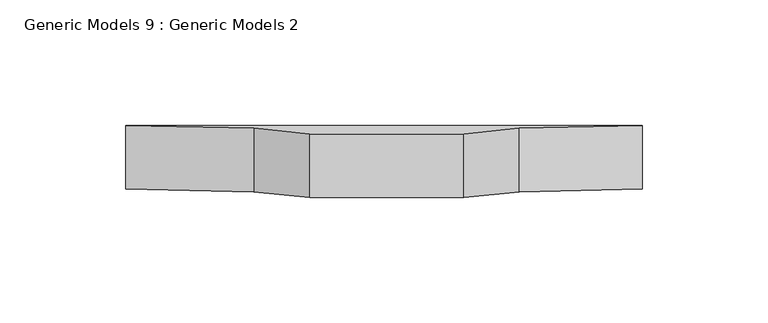
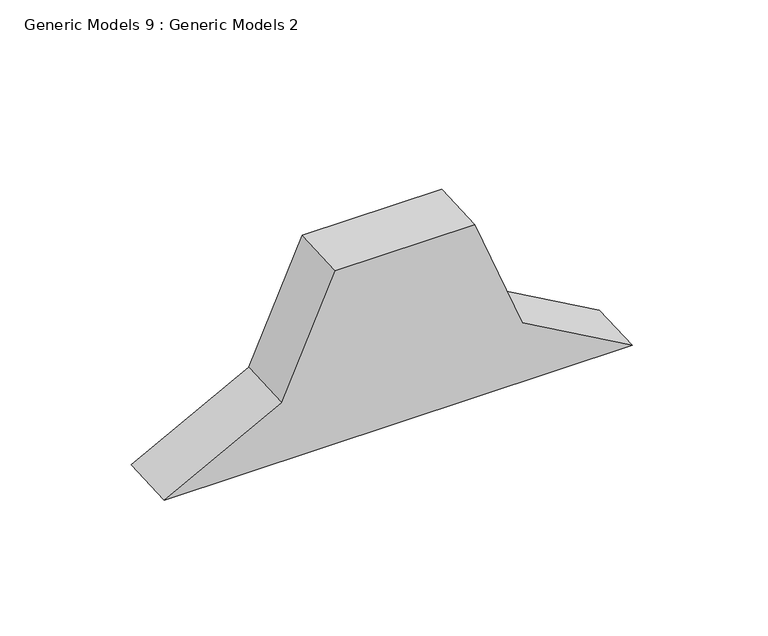
"""IFC4 building model written with IfcOpenShell, lengths in millimetres: proxy geometry, Generic Models 9 : Generic Models 2."""

from ifc_helpers import new_model, si_unit, frame, origin, place, context, project, spatial, polyline, outline, extrude, source, transform, mapped, element, save


def generic_models_9_generic_models_2_ba6f7f09(model_context):
    return source(origin(), model_context, "Body", "SweptSolid", [
        extrude(outline(polyline([(-38.6882115, -1e-07), (19.669451, 0.0), (-160.5378468, -99.7408183), (-131.3348102, -51.2109659), (-138.5264806, 7.6691636), (-84.8134897, 37.3981354), (-38.6882115, -1e-07)])), frame((592834.8996639, -568250.1646028, 8801.0491537), z_axis=(0.0, 0.9991330730923521, 0.041630544712176844), x_axis=(-0.8749277528680922, 0.02015973590912637, -0.48383366181908516)), (0.0, 0.0, 1.0), 25.4),
    ])


if __name__ == "__main__":
    model = new_model("IFC4")
    model_context = context("Model", 3, world=origin())
    ifc_project = project(units=[si_unit("LENGTHUNIT", "METRE", prefix="MILLI")], contexts=[model_context])
    site = spatial("IfcSite", under=ifc_project)
    building = spatial("IfcBuilding", under=site)
    placement = place(None, origin())
    generic_models_9_generic_models_2_shape = generic_models_9_generic_models_2_ba6f7f09(model_context)
    element("IfcBuildingElementProxy", 1, Name="Generic Models 9 : Generic Models 2", ObjectType="Generic Models 9 : Generic Models 2", at=placement, inside=building, context=model_context, shape_type="MappedRepresentation", body=[
        mapped(generic_models_9_generic_models_2_shape, transform((0.0, 0.0, 0.0), x_axis=(1.0, 0.0, 0.0), y_axis=(0.0, 1.0, 0.0), z_axis=(0.0, 0.0, 1.0))),
    ])
    save(model, "model.ifc")

# Revit data of these elements
# Element 1 (IfcBuildingElementProxy, "Generic Models 9 : Generic Models 2")
#   Materials on its faces: "METAL CLOSURE AT RIBS AND JOINTS - TAPE SEALER ALONG PERIMETER"
# Materials
#   "METAL CLOSURE AT RIBS AND JOINTS - TAPE SEALER ALONG PERIMETER": class "Generic", colour RGB 117 119 119, transparency 0, Cost = 0
